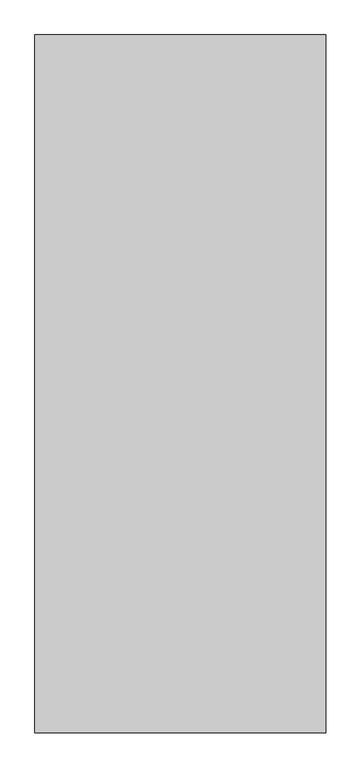
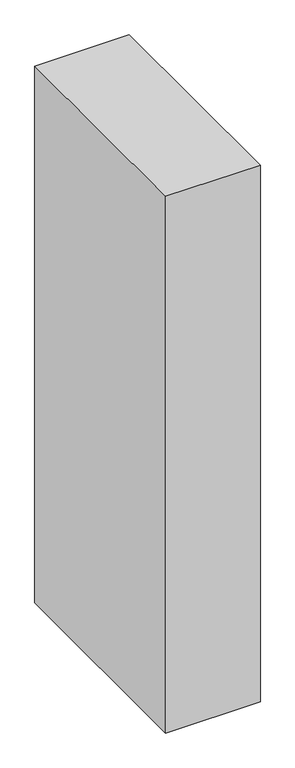
"""IFC4 building model written with IfcOpenShell, lengths in millimetres: proxy geometry, Space Planning Box_hec : Space Planning Box_hec."""

from ifc_helpers import new_model, si_unit, origin, origin_with_axes, place, context, project, spatial, polyline, outline, extrude, source, transform, mapped, element, save


def generic_models_21888712(model_context):
    return source(origin(), model_context, "Body", "SweptSolid", [
        extrude(outline(polyline([(500.0, 1200.0), (500.0, -1200.0), (-500.0, -1200.0), (-500.0, 1200.0), (500.0, 1200.0)])), origin_with_axes(), (0.0, 0.0, 1.0), 6000.0),
    ])


if __name__ == "__main__":
    model = new_model("IFC4")
    model_context = context("Model", 3, world=origin())
    ifc_project = project(units=[si_unit("LENGTHUNIT", "METRE", prefix="MILLI")], contexts=[model_context])
    site = spatial("IfcSite", under=ifc_project)
    building = spatial("IfcBuilding", under=site)
    placement = place(None, origin())
    generic_models_shape = generic_models_21888712(model_context)
    element("IfcBuildingElementProxy", 1, Name="Space Planning Box_hec : Space Planning Box_hec", ObjectType="Space Planning Box_hec : Space Planning Box_hec", at=placement, inside=building, context=model_context, shape_type="MappedRepresentation", body=[
        mapped(generic_models_shape, transform((0.0, 0.0, 0.0), x_axis=(1.0, 0.0, 0.0), y_axis=(0.0, 1.0, 0.0), z_axis=(0.0, 0.0, 1.0))),
    ])
    save(model, "model.ifc")

# Revit data of these elements
# Type "Space Planning Box_hec : Space Planning Box_hec"
#   Type Comments = "..."
#   Room Name [instance default] = "?"
#   Interior Finish [instance default] = ""
#   Exterior Finish [instance default] = ""
#   Department [instance default] = ""
#   Assembly Code = "..."
#   Width [instance default] = 1524 mm
#   Program Area [instance default] = 0.00 m²
#   Length [instance default] = 1524 mm
#   Height [instance default] = 1524 mm
#   Area [instance default] = 2.32258 m²
#   Fill Color [instance default] = Cyan
#   Default Elevation = 0
# Element 1 (IfcBuildingElementProxy, "Space Planning Box_hec : Space Planning Box_hec")
#   Room Name = "Pipe Shaft"
#   Interior Finish = "NA"
#   Exterior Finish = "EF1"
#   Department = "HV"
#   Width = 1000 mm
#   Program Area = 2.50 m²
#   Length = 2400 mm
#   Height = 6000 mm
#   Area = 2.40 m²
#   Fill Color = Pink
#   Materials on its faces: "Pink"
# Materials
#   "Cyan": class "Generic", colour RGB 0 255 255, transparency 0.2, Cost = 0
#   "Pink": class "Generic", colour RGB 255 105 180, transparency 0.2, Cost = 0
